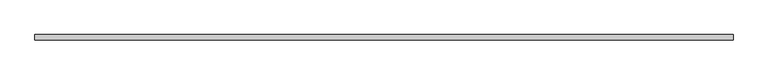
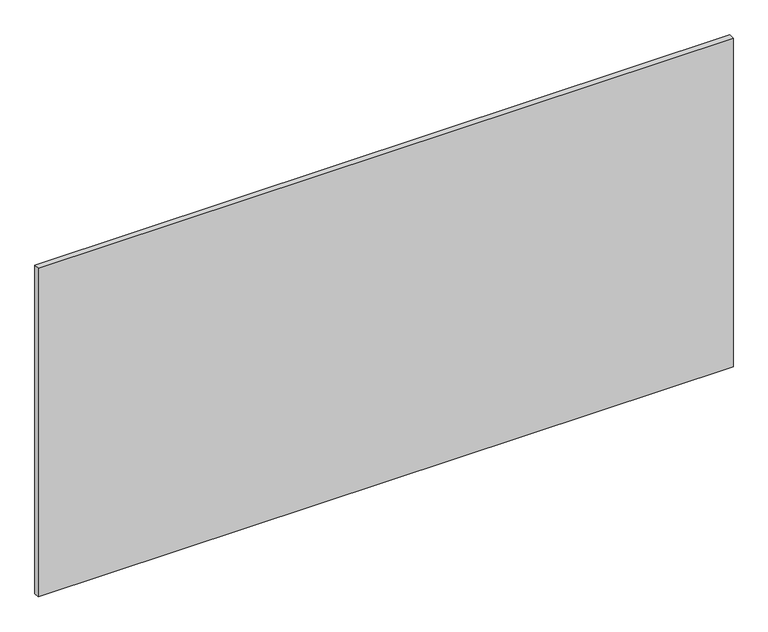
"""IFC4 building model written with IfcOpenShell, lengths in millimetres: proxy geometry, Inner panel:Inner panel:1:Inner panel:1 : Inner panel:Inner panel:300324:300043:Inner panel:1:Inner panel:1 : Inner panel:Inner panel:300324:300043 : Inner panel:Inner panel:1:Inner panel:1 : Inner panel:Inner panel:300324:300043:16 : Inner panel:Inner panel:1:Inner panel:1 : Inner panel:Inner panel:300324:300043:Inner panel:1:Inner panel:1 : Inner panel:Inner panel:300324:300043 : Inner panel:Inner panel:1:Inner panel:1 : Inner panel:Inner panel:300324:300043:300031."""

from ifc_helpers import new_model, si_unit, frame, origin, place, context, project, spatial, polyline, outline, extrude, source, transform, mapped, element, save


def generic_models_6113f932(model_context):
    return source(origin(), model_context, "Body", "SweptSolid", [
        extrude(outline(polyline([(570452.6367239, -578778.4413841), (572891.0367239, -578778.4413841), (572891.0367239, -578797.4913841), (570452.6367239, -578797.4913841), (570452.6367239, -578778.4413841)])), frame((0.0, 0.0, 2495.55), z_axis=(0.0, 0.0, 1.0), x_axis=(1.0, 0.0, 0.0)), (0.0, 0.0, 1.0), 1219.2),
    ])


if __name__ == "__main__":
    model = new_model("IFC4")
    model_context = context("Model", 3, world=origin())
    ifc_project = project(units=[si_unit("LENGTHUNIT", "METRE", prefix="MILLI")], contexts=[model_context])
    site = spatial("IfcSite", under=ifc_project)
    building = spatial("IfcBuilding", under=site)
    placement = place(None, origin())
    generic_models_shape = generic_models_6113f932(model_context)
    element("IfcBuildingElementProxy", 1, Name="Inner panel:Inner panel:1:Inner panel:1 : Inner panel:Inner panel:300324:300043:Inner panel:1:Inner panel:1 : Inner panel:Inner panel:300324:300043 : Inner panel:Inner panel:1:Inner panel:1 : Inner panel:Inner panel:300324:300043:16 : Inner panel:Inner panel:1:Inner panel:1 : Inner panel:Inner panel:300324:300043:Inner panel:1:Inner panel:1 : Inner panel:Inner panel:300324:300043 : Inner panel:Inner panel:1:Inner panel:1 : Inner panel:Inner panel:300324:300043:300031", ObjectType="Inner panel:Inner panel:1:Inner panel:1 : Inner panel:Inner panel:300324:300043:Inner panel:1:Inner panel:1 : Inner panel:Inner panel:300324:300043 : Inner panel:Inner panel:1:Inner panel:1 : Inner panel:Inner panel:300324:300043:16 : Inner panel:Inner panel:1:Inner panel:1 : Inner panel:Inner panel:300324:300043:Inner panel:1:Inner panel:1 : Inner panel:Inner panel:300324:300043 : Inner panel:Inner panel:1:Inner panel:1 : Inner panel:Inner panel:300324:300043:300031", at=placement, inside=building, context=model_context, shape_type="MappedRepresentation", body=[
        mapped(generic_models_shape, transform((0.0, 0.0, 0.0), x_axis=(1.0, 0.0, 0.0), y_axis=(0.0, 1.0, 0.0), z_axis=(0.0, 0.0, 1.0))),
    ])
    save(model, "model.ifc")

# Revit data of these elements
# Type "Inner panel:Inner panel:1:Inner panel:1 : Inner panel:Inner panel:300324:300043:Inner panel:1:Inner panel:1 : Inner panel:Inner panel:300324:300043 : Inner panel:Inner panel:1:Inner panel:1 : Inner panel:Inner panel:300324:300043:16 : Inner panel:Inner panel:1:Inner panel:1 : Inner panel:Inner panel:300324:300043:Inner panel:1:Inner panel:1 : Inner panel:Inner panel:300324:300043 : Inner panel:Inner panel:1:Inner panel:1 : Inner panel:Inner panel:300324:300043:300031"
#   NameOverride = "Inner panel:Inner panel:1:Inner panel:1 : Inner panel:Inner panel:300324:300043:Inner panel:1:Inner panel:1 : Inner panel:Inner panel:300324:300043 : Inner panel:Inner panel:1:Inner panel:1 : Inner panel:Inner panel:300324:300043:300031"
#   ObjectTypeOverride = "Inner panel:1:Inner panel:1 : Inner panel:Inner panel:300324:300043 : Inner panel:Inner panel:1:Inner panel:1 : Inner panel:Inner panel:300324:300043"
#   Reference = "Inner panel"
#   Tag = "300031"
# Element 1 (IfcBuildingElementProxy, "Inner panel:Inner panel:1:Inner panel:1 : Inner panel:Inner panel:300324:300043:Inner panel:1:Inner panel:1 : Inner panel:Inner panel:300324:300043 : Inner panel:Inner panel:1:Inner panel:1 : Inner panel:Inner panel:300324:300043:16 : Inner panel:Inner panel:1:Inner panel:1 : Inner panel:Inner panel:300324:300043:Inner panel:1:Inner panel:1 : Inner panel:Inner panel:300324:300043 : Inner panel:Inner panel:1:Inner panel:1 : Inner panel:Inner panel:300324:300043:300031")
#   Materials on its faces: "¾” (CLASS A) FIRE RETARDANT PLYWOOD ...OR… IF 1/4\" GYP. BD UNDER PLYWOOD, FLAME SPREAD TO BE CLASS C -  (FINISH: GRADE B - PREFINISHED STAINED/SEALED) - 1/4\" GAP BTWN PANELS (FASTENERS T.B.D.)"
# Materials
#   "¾” (CLASS A) FIRE RETARDANT PLYWOOD ...OR… IF 1/4\" GYP. BD UNDER PLYWOOD, FLAME SPREAD TO BE CLASS C -  (FINISH: GRADE B - PREFINISHED STAINED/SEALED) - 1/4\" GAP BTWN PANELS (FASTENERS T.B.D.)": class "Wood", colour RGB 149 120 74, transparency 0, Description = "Plywood, sheathing grade", Cost = 0
